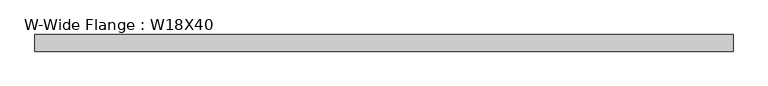
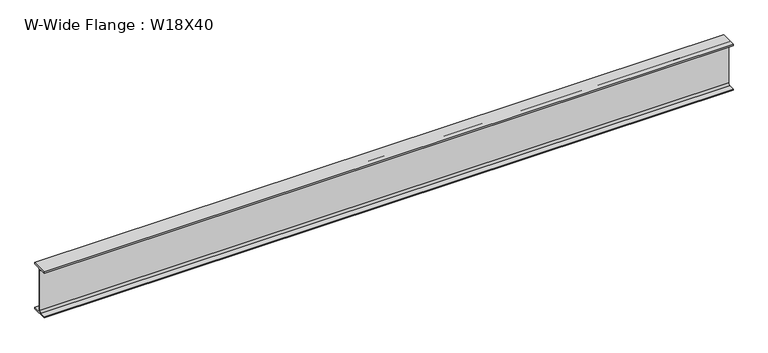
"""IFC4 building model written with IfcOpenShell, lengths in millimetres: beam geometry, W-Wide Flange : W18X40."""

from ifc_helpers import new_model, si_unit, point, frame, frame_2d, origin, place, context, project, spatial, polyline, circle_curve, trimmed, segment, composite_curve, outline, extrude, source, transform, mapped, element, save


def w_wide_flange_w18x40_7ff5a7d7(model_context):
    return source(origin(), model_context, "Body", "SweptSolid", [
        extrude(outline(composite_curve([segment(polyline([(76.454, -213.995), (76.454, -227.33), (-76.454, -227.33), (-76.454, -213.995), (-20.828, -213.995)]), True, "CONTINUOUS"), segment(trimmed(circle_curve(frame_2d((-20.828, -197.1675)), 16.8275), [point((-20.828, -213.995))], [point((-4.0005, -197.1675))], True, "CARTESIAN"), True, "CONTINUOUS"), segment(polyline([(-4.0005, -197.1675), (-4.0005, 197.1675)]), True, "CONTINUOUS"), segment(trimmed(circle_curve(frame_2d((-20.828, 197.1675)), 16.8275), [point((-4.0005, 197.1675))], [point((-20.828, 213.995))], True, "CARTESIAN"), True, "CONTINUOUS"), segment(polyline([(-20.828, 213.995), (-76.454, 213.995), (-76.454, 227.33), (76.454, 227.33), (76.454, 213.995), (20.828, 213.995)]), True, "CONTINUOUS"), segment(trimmed(circle_curve(frame_2d((20.828, 197.1675)), 16.8275), [point((20.828, 213.995))], [point((4.0005, 197.1675))], True, "CARTESIAN"), True, "CONTINUOUS"), segment(polyline([(4.0005, 197.1675), (4.0005, -197.1675)]), True, "CONTINUOUS"), segment(trimmed(circle_curve(frame_2d((20.828, -197.1675)), 16.8275), [point((4.0005, -197.1675))], [point((20.828, -213.995))], True, "CARTESIAN"), True, "CONTINUOUS"), segment(polyline([(20.828, -213.995), (76.454, -213.995)]), True, "CONTINUOUS")], self_intersect=False)), frame((-3211.83, 0.0, 0.0), z_axis=(1.0, 0.0, 0.0), x_axis=(0.0, 1.0, 0.0)), (0.0, 0.0, 1.0), 6423.66),
    ])


if __name__ == "__main__":
    model = new_model("IFC4")
    model_context = context("Model", 3, world=origin())
    ifc_project = project(units=[si_unit("LENGTHUNIT", "METRE", prefix="MILLI")], contexts=[model_context])
    site = spatial("IfcSite", under=ifc_project)
    building = spatial("IfcBuilding", under=site)
    placement = place(None, origin())
    w_wide_flange_w18x40_shape = w_wide_flange_w18x40_7ff5a7d7(model_context)
    element("IfcBeam", 1, ObjectType="W-Wide Flange : W18X40", at=placement, inside=building, context=model_context, shape_type="MappedRepresentation", body=[
        mapped(w_wide_flange_w18x40_shape, transform((0.0, 0.0, 0.0), x_axis=(1.0, 0.0, 0.0), y_axis=(0.0, 1.0, 0.0), z_axis=(0.0, 0.0, 1.0))),
    ])
    save(model, "model.ifc")

# Revit data of these elements
# Type "W-Wide Flange : W18X40"
#   Assembly Code = "B10"
#   W = 40
#   Length [instance default] = 5' - 0"
#   bf = 0' - 6.02"
#   d = 1' - 5.9"
#   k = 0' - 1 3/16"
#   k2 = 0' - 0.6625"
#   tf = 0' - 0.525"
#   tw = 0' - 0.315"
#   A = 0.0819444 SF
#   Structural Material [instance default] = Steel ASTM A992
# Element 1 (IfcBeam, "W-Wide Flange : W18X40")
#   Materials on its faces: "Steel ASTM A992"
# Materials
#   "Steel ASTM A992": class "Metal", colour RGB 199 199 199, transparency 0, Description = "Structural steel 50ksi", Cost = 0
